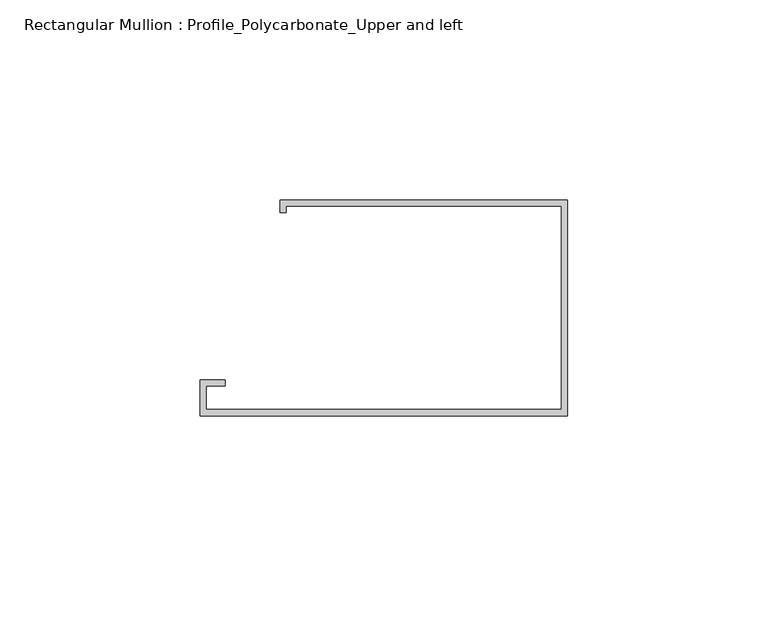
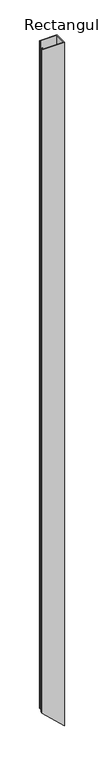
"""IFC4 building model written with IfcOpenShell, lengths in millimetres: member geometry, Rectangular Mullion : Profile_Polycarbonate_Upper and left."""

from ifc_helpers import new_model, si_unit, origin, place, context, project, spatial, faceted_brep, source, transform, mapped, element, save


def rectangular_mullion_profile_polycarbonate_upper_and_left_1557256d(model_context):
    return source(origin(), model_context, "Body", "Brep", [
        faceted_brep([(0.0, -28.984575, 0.0), (0.0, 25.015825, 0.0), (-71.9836, 25.015825, 0.0), (-71.9836, 21.840825, 0.0), (-70.3961, 21.840825, 0.0), (-70.3961, 23.428325, 0.0), (-1.5875, 23.428325, 0.0), (-1.5875, -27.397075, 0.0), (-90.4113, -27.397075, 0.0), (-90.4113, -21.580475, 0.0), (-85.6488, -21.580475, 0.0), (-85.6488, -19.992975, 0.0), (-91.9988, -19.992975, 0.0), (-91.9988, -28.984575, 0.0), (0.0, -28.984575, -3006.4840978), (0.0, 25.015825, -3006.4840978), (-71.9836, 25.015825, -2937.4373558), (-71.9836, 21.840825, -2937.4373558), (-70.3961, 21.840825, -2938.9600874), (-70.3961, 23.428325, -2938.9600874), (-1.5875, 23.428325, -3004.9613662), (-1.5875, -27.397075, -3004.9613662), (-90.4113, -27.397075, -2919.7614873), (-90.4113, -21.580475, -2919.7614873), (-85.6488, -21.580475, -2924.3296821), (-85.6488, -19.992975, -2924.3296821), (-91.9988, -19.992975, -2918.2387557), (-91.9988, -28.984575, -2918.2387557)], [[[0, 1, 2, 3, 4, 5, 6, 7, 8, 9, 10, 11, 12, 13]], [[1, 0, 14, 15]], [[2, 1, 15, 16]], [[3, 2, 16, 17]], [[4, 3, 17, 18]], [[5, 4, 18, 19]], [[6, 5, 19, 20]], [[7, 6, 20, 21]], [[8, 7, 21, 22]], [[9, 8, 22, 23]], [[10, 9, 23, 24]], [[11, 10, 24, 25]], [[12, 11, 25, 26]], [[13, 12, 26, 27]], [[0, 13, 27, 14]], [[14, 27, 26, 25, 24, 23, 22, 21, 20, 19, 18, 17, 16, 15]]]),
    ])


if __name__ == "__main__":
    model = new_model("IFC4")
    model_context = context("Model", 3, world=origin())
    ifc_project = project(units=[si_unit("LENGTHUNIT", "METRE", prefix="MILLI")], contexts=[model_context])
    site = spatial("IfcSite", under=ifc_project)
    building = spatial("IfcBuilding", under=site)
    placement = place(None, origin())
    rectangular_mullion_profile_polycarbonate_upper_and_left_shape = rectangular_mullion_profile_polycarbonate_upper_and_left_1557256d(model_context)
    element("IfcMember", 1, ObjectType="Rectangular Mullion : Profile_Polycarbonate_Upper and left", at=placement, inside=building, context=model_context, shape_type="MappedRepresentation", body=[
        mapped(rectangular_mullion_profile_polycarbonate_upper_and_left_shape, transform((0.0, 0.0, 0.0), x_axis=(1.0, 0.0, 0.0), y_axis=(0.0, 1.0, 0.0), z_axis=(0.0, 0.0, 1.0))),
    ])
    save(model, "model.ifc")

# Revit data of these elements
# Type "Rectangular Mullion : Profile_Polycarbonate_Upper and left"
#   built-in parameter 1007322 = 0.177167 (stored number, unit not read)
#   built-in parameter 1007321 = 0.00520833 (stored number, unit not read)
#   built-in parameter 1007320 = 0 (stored number, unit not read)
